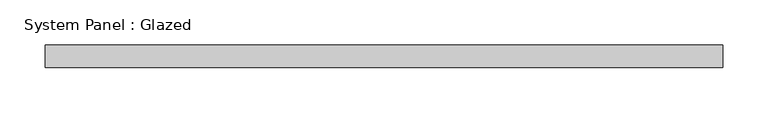
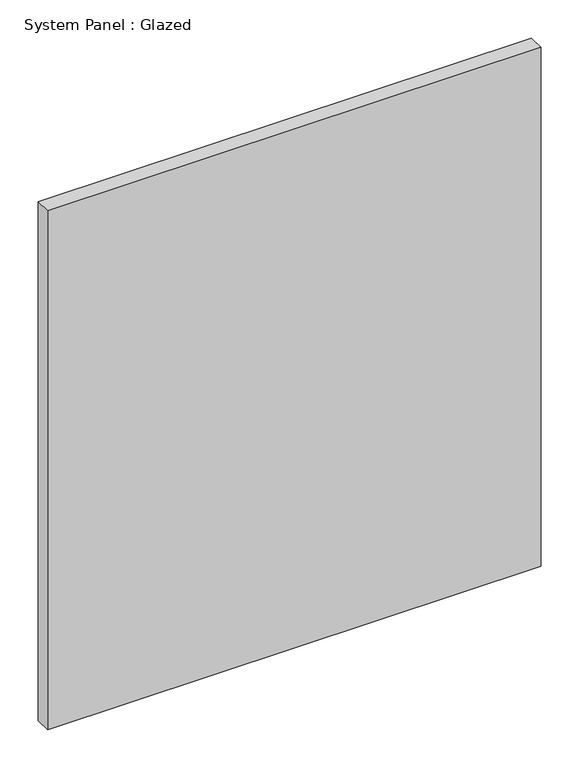
"""IFC4 building model written with IfcOpenShell, lengths in millimetres: plate geometry, System Panel : Glazed."""

import ifcopenshell
import ifcopenshell.guid

model = None  # the IFC model being written
_history = None  # IfcOwnerHistory: only IFC2X3 demands one
_inside = {}  # id of a spatial element -> (the spatial element, [elements in it])
_under = {}  # id of a project, library or spatial element -> (it, [spatial elements below it])
_declared = {}  # id of a project -> (the project, [libraries it declares])
_typed = {}  # id of a type object -> (the type object, [elements of that type])
_made_of = {}  # id of a material, layer set ... -> (it, [elements and type objects made of it])


def new_model(schema):
    """Start an empty IFC model of exactly this schema.

    Asked for "IFC4X3", IfcOpenShell would pick the latest addendum, in which some entities
    have other attributes; the version numbers below select the first issue.
    IFC2X3 requires an IfcOwnerHistory on every rooted entity: one is made here for all.
    """
    global model, _history
    if schema == "IFC4X3":
        model = ifcopenshell.file(schema_version=(4, 3, 0, 0))
    else:
        model = ifcopenshell.file(schema=schema)
    _inside.clear()
    _under.clear()
    _declared.clear()
    _typed.clear()
    _made_of.clear()
    _history = None
    if model.schema == "IFC2X3":
        org = make("IfcOrganization", Name="unknown")
        user = make(
            "IfcPersonAndOrganization",
            ThePerson=make("IfcPerson", FamilyName="unknown"),
            TheOrganization=org,
        )
        app = make(
            "IfcApplication",
            ApplicationDeveloper=org,
            Version="unknown",
            ApplicationFullName="unknown",
            ApplicationIdentifier="unknown",
        )
        _history = make(
            "IfcOwnerHistory",
            OwningUser=user,
            OwningApplication=app,
            ChangeAction="ADDED",
            CreationDate=0,
        )
    return model


def make(cls, **values):
    """One entity of the class cls with the attributes given. An attribute that is None is left unset."""
    return model.create_entity(
        cls, **{name: value for name, value in values.items() if value is not None}
    )


def rooted(cls, **values):
    """An entity with a GlobalId (a new one), such as an element, a storey or a relation."""
    return make(cls, GlobalId=ifcopenshell.guid.new(), OwnerHistory=_history, **values)


def si_unit(unit_type, name, prefix=None):
    """IfcSIUnit, for example si_unit("LENGTHUNIT", "METRE", prefix="MILLI")."""
    return make("IfcSIUnit", UnitType=unit_type, Prefix=prefix, Name=name)


def assignment(units):
    """IfcUnitAssignment: the units of a project."""
    return None if units is None else make("IfcUnitAssignment", Units=units)


def point(xyz):
    """IfcCartesianPoint."""
    return None if xyz is None else make("IfcCartesianPoint", Coordinates=xyz)


def direction(xyz):
    """IfcDirection."""
    return None if xyz is None else make("IfcDirection", DirectionRatios=xyz)


def frame(location, z_axis=None, x_axis=None):
    """IfcAxis2Placement3D, a coordinate frame: its origin and axes. An axis left out is left unset."""
    return make(
        "IfcAxis2Placement3D",
        Location=point(location),
        Axis=direction(z_axis),
        RefDirection=direction(x_axis),
    )


def origin():
    """The frame at (0, 0, 0) with its axes left unset."""
    return frame((0.0, 0.0, 0.0))


def origin_with_axes():
    """The frame at (0, 0, 0) with the z axis (0, 0, 1) and the x axis (1, 0, 0) written out."""
    return frame((0.0, 0.0, 0.0), z_axis=(0.0, 0.0, 1.0), x_axis=(1.0, 0.0, 0.0))


def place(relative_to, where):
    """IfcLocalPlacement: puts the frame where relative to a parent placement (None: the world)."""
    return make(
        "IfcLocalPlacement", PlacementRelTo=relative_to, RelativePlacement=where
    )


def context(
    kind, dimensions, precision=None, world=None, true_north=None, identifier=None
):
    """IfcGeometricRepresentationContext, for example the 3D "Model" context."""
    return make(
        "IfcGeometricRepresentationContext",
        ContextIdentifier=identifier,
        ContextType=kind,
        CoordinateSpaceDimension=dimensions,
        Precision=precision,
        WorldCoordinateSystem=world,
        TrueNorth=true_north,
    )


def project(units=None, contexts=None):
    """IfcProject with its units and contexts."""
    return rooted(
        "IfcProject",
        Name="project",
        RepresentationContexts=contexts,
        UnitsInContext=assignment(units),
    )


def spatial(cls, under=None, at=None, **own):
    """A site, building, storey or space (cls), placed at a placement, below another one or the project."""
    s = rooted(cls, ObjectPlacement=at, **own)
    if under is not None:
        _under.setdefault(under.id(), (under, []))[1].append(s)
    return s


def polyline(points):
    """IfcPolyline through the points."""
    return make("IfcPolyline", Points=[point(p) for p in points])


def outline(outer, holes=None, kind="AREA"):
    """IfcArbitraryClosedProfileDef: a profile drawn as a closed curve; with holes, ...WithVoids."""
    if holes is None:
        return make("IfcArbitraryClosedProfileDef", ProfileType=kind, OuterCurve=outer)
    return make(
        "IfcArbitraryProfileDefWithVoids",
        ProfileType=kind,
        OuterCurve=outer,
        InnerCurves=holes,
    )


def extrude(swept, where, along, depth):
    """IfcExtrudedAreaSolid: the profile swept, set in the frame where, extruded along a direction by depth."""
    return make(
        "IfcExtrudedAreaSolid",
        SweptArea=swept,
        Position=where,
        ExtrudedDirection=direction(along),
        Depth=depth,
    )


def shape(context_of_items, identifier, shape_type, items):
    """IfcShapeRepresentation: the items that make up one representation, for example the "Body"."""
    return make(
        "IfcShapeRepresentation",
        ContextOfItems=context_of_items,
        RepresentationIdentifier=identifier,
        RepresentationType=shape_type,
        Items=items,
    )


def source(mapping_origin, context_of_items, identifier, shape_type, items):
    """IfcRepresentationMap: a shape defined once, which mapped items show again and again."""
    return make(
        "IfcRepresentationMap",
        MappingOrigin=mapping_origin,
        MappedRepresentation=shape(context_of_items, identifier, shape_type, items),
    )


def transform(
    local_origin,
    x_axis=None,
    y_axis=None,
    z_axis=None,
    scale=None,
    scale2=None,
    scale3=None,
    uniform=True,
):
    """IfcCartesianTransformationOperator3D, or its non-uniform kind. x_axis, y_axis, z_axis: its Axis1, 2, 3."""
    if uniform:
        return make(
            "IfcCartesianTransformationOperator3D",
            Axis1=direction(x_axis),
            Axis2=direction(y_axis),
            LocalOrigin=point(local_origin),
            Scale=scale,
            Axis3=direction(z_axis),
        )
    return make(
        "IfcCartesianTransformationOperator3DnonUniform",
        Axis1=direction(x_axis),
        Axis2=direction(y_axis),
        LocalOrigin=point(local_origin),
        Scale=scale,
        Axis3=direction(z_axis),
        Scale2=scale2,
        Scale3=scale3,
    )


def mapped(mapping_source, mapping_target):
    """IfcMappedItem: shows the shape of a source again, moved by a transform."""
    return make(
        "IfcMappedItem", MappingSource=mapping_source, MappingTarget=mapping_target
    )


def made_of(thing, what):
    """Note that an element or type object is made of a material, layer set ...; save() writes the relation."""
    if what is not None:
        _made_of.setdefault(what.id(), (what, []))[1].append(thing)
    return thing


def element(
    cls,
    number,
    at=None,
    inside=None,
    cuts=None,
    type_object=None,
    material=None,
    context=None,
    identifier="Body",
    shape_type=None,
    held_by="IfcProductDefinitionShape",
    body=None,
    shapes=None,
    **own,
):
    """One element of the class cls, such as IfcWall. Its Tag is "e" and its number.

    at: its placement. inside: the storey or other place that contains it. cuts: it is an
    opening in that element (IfcRelVoidsElement). A single representation is given by context,
    identifier, shape_type and body (its items); several are given by shapes. held_by: the class
    of the entity that holds the representations. save() writes the other relations.
    """
    e = rooted(cls, Tag="e%d" % number, ObjectPlacement=at, **own)
    if body is not None:
        shapes = [shape(context, identifier, shape_type, body)]
    if shapes is not None:
        e.Representation = make(held_by, Representations=shapes)
    if inside is not None:
        _inside.setdefault(inside.id(), (inside, []))[1].append(e)
    if cuts is not None:
        rooted(
            "IfcRelVoidsElement", RelatingBuildingElement=cuts, RelatedOpeningElement=e
        )
    if type_object is not None:
        _typed.setdefault(type_object.id(), (type_object, []))[1].append(e)
    return made_of(e, material)


def aggregate(whole, parts):
    """IfcRelAggregates: a whole, such as a stair, and the parts it consists of."""
    return rooted("IfcRelAggregates", RelatingObject=whole, RelatedObjects=parts)


def save(model, path):
    """Write the relations noted so far, then the file.

    IfcRelAggregates (storeys below a building ...), IfcRelContainedInSpatialStructure (elements
    in a storey), IfcRelDefinesByType, IfcRelAssociatesMaterial and IfcRelDeclares: one each for
    every whole, place, type object, material and project.
    """
    for whole, parts in _under.values():
        aggregate(whole, parts)
    for where, things in _inside.values():
        rooted(
            "IfcRelContainedInSpatialStructure",
            RelatedElements=things,
            RelatingStructure=where,
        )
    for kind, things in _typed.values():
        rooted("IfcRelDefinesByType", RelatedObjects=things, RelatingType=kind)
    for what, things in _made_of.values():
        rooted("IfcRelAssociatesMaterial", RelatedObjects=things, RelatingMaterial=what)
    for by, libraries in _declared.values():
        rooted("IfcRelDeclares", RelatingContext=by, RelatedDefinitions=libraries)
    model.write(path)


def system_panel_glazed_ff5c23df(model_context):
    return source(origin(), model_context, "Body", "SweptSolid", [
        extrude(outline(polyline([(375.0, 24.5), (-375.0, 24.5), (-375.0, 49.5), (375.0, 49.5), (375.0, 24.5)])), origin_with_axes(), (0.0, 0.0, 1.0), 833.3333333),
    ])


if __name__ == "__main__":
    model = new_model("IFC4")
    model_context = context("Model", 3, world=origin())
    ifc_project = project(units=[si_unit("LENGTHUNIT", "METRE", prefix="MILLI")], contexts=[model_context])
    site = spatial("IfcSite", under=ifc_project)
    building = spatial("IfcBuilding", under=site)
    placement = place(None, origin())
    system_panel_glazed_shape = system_panel_glazed_ff5c23df(model_context)
    element("IfcPlate", 1, ObjectType="System Panel : Glazed", at=placement, inside=building, context=model_context, shape_type="MappedRepresentation", body=[
        mapped(system_panel_glazed_shape, transform((0.0, 0.0, 0.0), x_axis=(1.0, 0.0, 0.0), y_axis=(0.0, 1.0, 0.0), z_axis=(0.0, 0.0, 1.0))),
    ])
    save(model, "model.ifc")

# Revit data of these elements
# Element 1 (IfcPlate, "System Panel : Glazed")
#   Materials on its faces: "Glass"
# Materials
#   "Glass": class "Glass", colour RGB 218 227 224, transparency 0.85, Description = "Soda Lime Glass", Cost = 0
